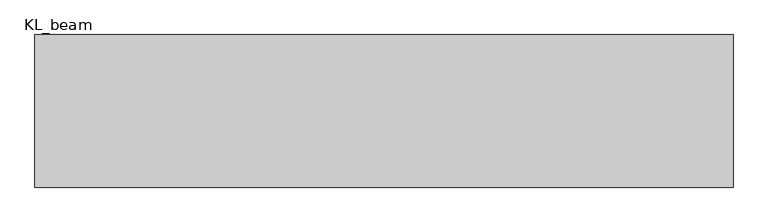
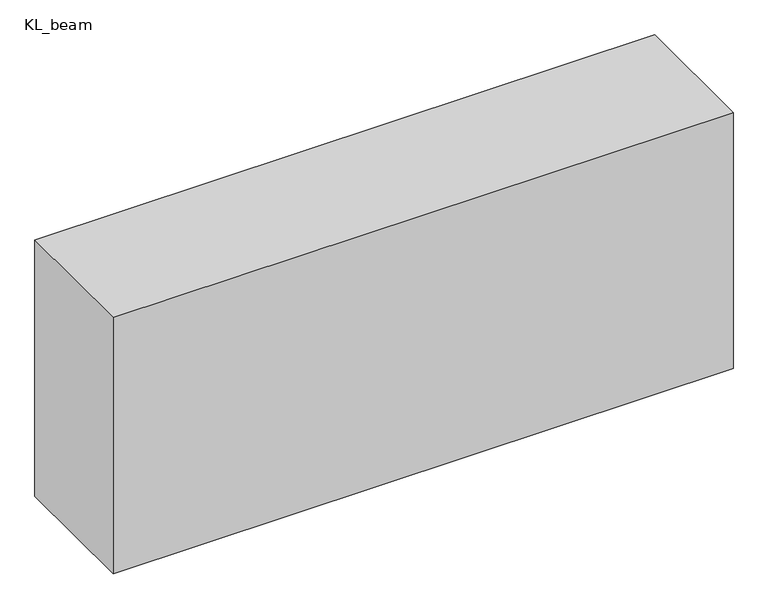
"""IFC4 building model written with IfcOpenShell, lengths in millimetres: beam geometry, 混凝土 - 矩形梁 : KL_beam."""

from ifc_helpers import new_model, si_unit, frame, origin, place, context, project, spatial, polyline, outline, extrude, source, transform, mapped, element, save


def kl_beam_00cea109(model_context):
    return source(origin(), model_context, "Body", "SweptSolid", [
        extrude(outline(polyline([(915.0, 200.0), (915.0, -200.0), (-915.0, -200.0), (-915.0, 200.0), (915.0, 200.0)])), frame((0.0, 0.0, -400.0), z_axis=(0.0, 0.0, 1.0), x_axis=(1.0, 0.0, 0.0)), (0.0, 0.0, 1.0), 800.0),
    ])


if __name__ == "__main__":
    model = new_model("IFC4")
    model_context = context("Model", 3, world=origin())
    ifc_project = project(units=[si_unit("LENGTHUNIT", "METRE", prefix="MILLI")], contexts=[model_context])
    site = spatial("IfcSite", under=ifc_project)
    building = spatial("IfcBuilding", under=site)
    placement = place(None, origin())
    kl_beam_shape = kl_beam_00cea109(model_context)
    element("IfcBeam", 1, ObjectType="混凝土 - 矩形梁 : KL_beam", at=placement, inside=building, context=model_context, shape_type="MappedRepresentation", body=[
        mapped(kl_beam_shape, transform((0.0, 0.0, 0.0), x_axis=(1.0, 0.0, 0.0), y_axis=(0.0, 1.0, 0.0), z_axis=(0.0, 0.0, 1.0))),
    ])
    save(model, "model.ifc")

# Revit data of these elements
# Type "混凝土 - 矩形梁 : KL_beam"
#   Length [instance default] = 1524 mm
#   b = 400 mm
#   h = 800 mm
#   Structural Material [instance default] = 混凝土 - 现场浇注混凝土
#   Assembly Code = ""
# Element 1 (IfcBeam, "混凝土 - 矩形梁 : KL_beam")
#   Structural Material = none
# Materials
#   "混凝土 - 现场浇注混凝土": class "混凝土", colour RGB 192 192 192, transparency 0
